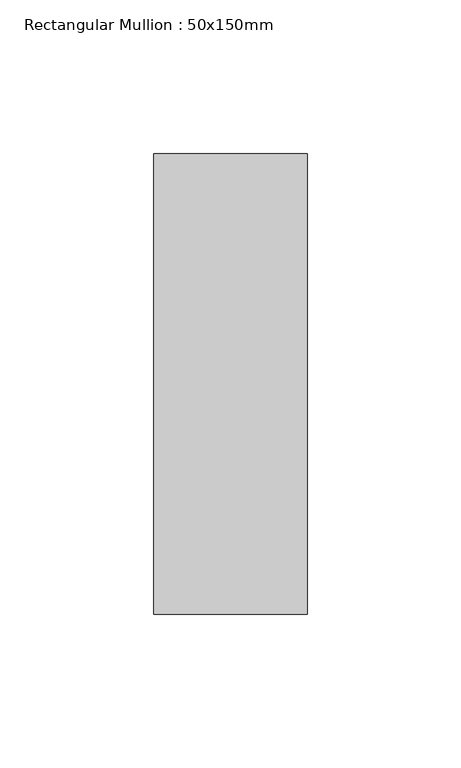
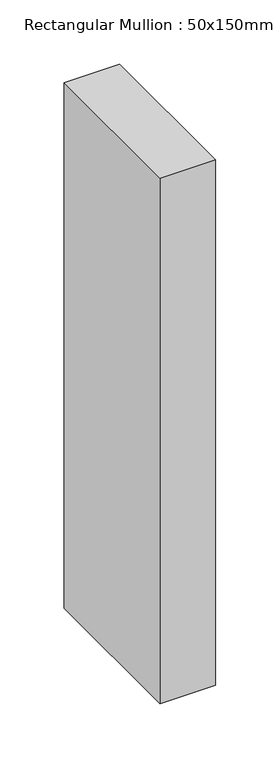
"""IFC4 building model written with IfcOpenShell, lengths in millimetres: member geometry, Rectangular Mullion : 50x150mm."""

from ifc_helpers import new_model, si_unit, frame, origin, place, context, project, spatial, polyline, outline, extrude, source, transform, mapped, element, save


def rectangular_mullion_50x150mm_b3666dbd(model_context):
    return source(origin(), model_context, "Body", "SweptSolid", [
        extrude(outline(polyline([(0.0, 75.0), (0.0, -75.0), (-50.0, -75.0), (-50.0, 75.0), (0.0, 75.0)])), frame((0.0, 0.0, -500.0), z_axis=(0.0, 0.0, 1.0), x_axis=(1.0, 0.0, 0.0)), (0.0, 0.0, 1.0), 500.0),
    ])


if __name__ == "__main__":
    model = new_model("IFC4")
    model_context = context("Model", 3, world=origin())
    ifc_project = project(units=[si_unit("LENGTHUNIT", "METRE", prefix="MILLI")], contexts=[model_context])
    site = spatial("IfcSite", under=ifc_project)
    building = spatial("IfcBuilding", under=site)
    placement = place(None, origin())
    rectangular_mullion_50x150mm_shape = rectangular_mullion_50x150mm_b3666dbd(model_context)
    element("IfcMember", 1, ObjectType="Rectangular Mullion : 50x150mm", at=placement, inside=building, context=model_context, shape_type="MappedRepresentation", body=[
        mapped(rectangular_mullion_50x150mm_shape, transform((0.0, 0.0, 0.0), x_axis=(1.0, 0.0, 0.0), y_axis=(0.0, 1.0, 0.0), z_axis=(0.0, 0.0, 1.0))),
    ])
    save(model, "model.ifc")

# Revit data of these elements
# Type "Rectangular Mullion : 50x150mm"
#   Keynote = "H11"
#   built-in parameter 1007304 = 0.492126 (stored number, unit not read)
#   built-in parameter 1007301 = 0.082021 (stored number, unit not read)
#   built-in parameter 1007300 = 0.082021 (stored number, unit not read)
# Element 1 (IfcMember, "Rectangular Mullion : 50x150mm")
#   Materials on its faces: "Aluminium"
# Materials
#   "Aluminium": class "Metal", colour RGB 247 247 247, transparency 0, Description = "Aluminium 6061", Cost = 0
